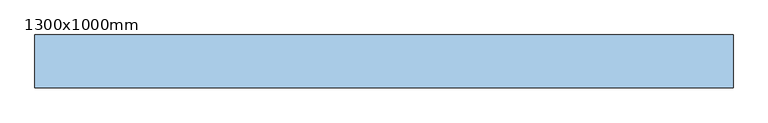
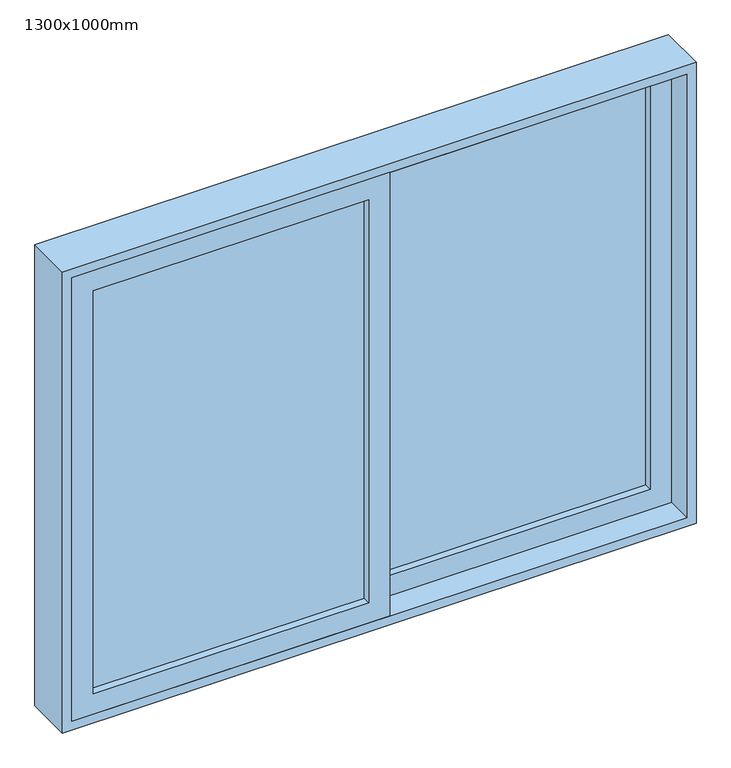
"""IFC4 building model written with IfcOpenShell, lengths in millimetres: window geometry, Janela de Correr - 2 Folhas : 1300x1000mm."""

import ifcopenshell
import ifcopenshell.guid

model = None  # the IFC model being written
_history = None  # IfcOwnerHistory: only IFC2X3 demands one
_inside = {}  # id of a spatial element -> (the spatial element, [elements in it])
_under = {}  # id of a project, library or spatial element -> (it, [spatial elements below it])
_declared = {}  # id of a project -> (the project, [libraries it declares])
_typed = {}  # id of a type object -> (the type object, [elements of that type])
_made_of = {}  # id of a material, layer set ... -> (it, [elements and type objects made of it])


def new_model(schema):
    """Start an empty IFC model of exactly this schema.

    Asked for "IFC4X3", IfcOpenShell would pick the latest addendum, in which some entities
    have other attributes; the version numbers below select the first issue.
    IFC2X3 requires an IfcOwnerHistory on every rooted entity: one is made here for all.
    """
    global model, _history
    if schema == "IFC4X3":
        model = ifcopenshell.file(schema_version=(4, 3, 0, 0))
    else:
        model = ifcopenshell.file(schema=schema)
    _inside.clear()
    _under.clear()
    _declared.clear()
    _typed.clear()
    _made_of.clear()
    _history = None
    if model.schema == "IFC2X3":
        org = make("IfcOrganization", Name="unknown")
        user = make(
            "IfcPersonAndOrganization",
            ThePerson=make("IfcPerson", FamilyName="unknown"),
            TheOrganization=org,
        )
        app = make(
            "IfcApplication",
            ApplicationDeveloper=org,
            Version="unknown",
            ApplicationFullName="unknown",
            ApplicationIdentifier="unknown",
        )
        _history = make(
            "IfcOwnerHistory",
            OwningUser=user,
            OwningApplication=app,
            ChangeAction="ADDED",
            CreationDate=0,
        )
    return model


def make(cls, **values):
    """One entity of the class cls with the attributes given. An attribute that is None is left unset."""
    return model.create_entity(
        cls, **{name: value for name, value in values.items() if value is not None}
    )


def rooted(cls, **values):
    """An entity with a GlobalId (a new one), such as an element, a storey or a relation."""
    return make(cls, GlobalId=ifcopenshell.guid.new(), OwnerHistory=_history, **values)


def si_unit(unit_type, name, prefix=None):
    """IfcSIUnit, for example si_unit("LENGTHUNIT", "METRE", prefix="MILLI")."""
    return make("IfcSIUnit", UnitType=unit_type, Prefix=prefix, Name=name)


def assignment(units):
    """IfcUnitAssignment: the units of a project."""
    return None if units is None else make("IfcUnitAssignment", Units=units)


def point(xyz):
    """IfcCartesianPoint."""
    return None if xyz is None else make("IfcCartesianPoint", Coordinates=xyz)


def direction(xyz):
    """IfcDirection."""
    return None if xyz is None else make("IfcDirection", DirectionRatios=xyz)


def frame(location, z_axis=None, x_axis=None):
    """IfcAxis2Placement3D, a coordinate frame: its origin and axes. An axis left out is left unset."""
    return make(
        "IfcAxis2Placement3D",
        Location=point(location),
        Axis=direction(z_axis),
        RefDirection=direction(x_axis),
    )


def origin():
    """The frame at (0, 0, 0) with its axes left unset."""
    return frame((0.0, 0.0, 0.0))


def place(relative_to, where):
    """IfcLocalPlacement: puts the frame where relative to a parent placement (None: the world)."""
    return make(
        "IfcLocalPlacement", PlacementRelTo=relative_to, RelativePlacement=where
    )


def context(
    kind, dimensions, precision=None, world=None, true_north=None, identifier=None
):
    """IfcGeometricRepresentationContext, for example the 3D "Model" context."""
    return make(
        "IfcGeometricRepresentationContext",
        ContextIdentifier=identifier,
        ContextType=kind,
        CoordinateSpaceDimension=dimensions,
        Precision=precision,
        WorldCoordinateSystem=world,
        TrueNorth=true_north,
    )


def project(units=None, contexts=None):
    """IfcProject with its units and contexts."""
    return rooted(
        "IfcProject",
        Name="project",
        RepresentationContexts=contexts,
        UnitsInContext=assignment(units),
    )


def spatial(cls, under=None, at=None, **own):
    """A site, building, storey or space (cls), placed at a placement, below another one or the project."""
    s = rooted(cls, ObjectPlacement=at, **own)
    if under is not None:
        _under.setdefault(under.id(), (under, []))[1].append(s)
    return s


def polyline(points):
    """IfcPolyline through the points."""
    return make("IfcPolyline", Points=[point(p) for p in points])


def outline(outer, holes=None, kind="AREA"):
    """IfcArbitraryClosedProfileDef: a profile drawn as a closed curve; with holes, ...WithVoids."""
    if holes is None:
        return make("IfcArbitraryClosedProfileDef", ProfileType=kind, OuterCurve=outer)
    return make(
        "IfcArbitraryProfileDefWithVoids",
        ProfileType=kind,
        OuterCurve=outer,
        InnerCurves=holes,
    )


def extrude(swept, where, along, depth):
    """IfcExtrudedAreaSolid: the profile swept, set in the frame where, extruded along a direction by depth."""
    return make(
        "IfcExtrudedAreaSolid",
        SweptArea=swept,
        Position=where,
        ExtrudedDirection=direction(along),
        Depth=depth,
    )


def shape(context_of_items, identifier, shape_type, items):
    """IfcShapeRepresentation: the items that make up one representation, for example the "Body"."""
    return make(
        "IfcShapeRepresentation",
        ContextOfItems=context_of_items,
        RepresentationIdentifier=identifier,
        RepresentationType=shape_type,
        Items=items,
    )


def source(mapping_origin, context_of_items, identifier, shape_type, items):
    """IfcRepresentationMap: a shape defined once, which mapped items show again and again."""
    return make(
        "IfcRepresentationMap",
        MappingOrigin=mapping_origin,
        MappedRepresentation=shape(context_of_items, identifier, shape_type, items),
    )


def transform(
    local_origin,
    x_axis=None,
    y_axis=None,
    z_axis=None,
    scale=None,
    scale2=None,
    scale3=None,
    uniform=True,
):
    """IfcCartesianTransformationOperator3D, or its non-uniform kind. x_axis, y_axis, z_axis: its Axis1, 2, 3."""
    if uniform:
        return make(
            "IfcCartesianTransformationOperator3D",
            Axis1=direction(x_axis),
            Axis2=direction(y_axis),
            LocalOrigin=point(local_origin),
            Scale=scale,
            Axis3=direction(z_axis),
        )
    return make(
        "IfcCartesianTransformationOperator3DnonUniform",
        Axis1=direction(x_axis),
        Axis2=direction(y_axis),
        LocalOrigin=point(local_origin),
        Scale=scale,
        Axis3=direction(z_axis),
        Scale2=scale2,
        Scale3=scale3,
    )


def mapped(mapping_source, mapping_target):
    """IfcMappedItem: shows the shape of a source again, moved by a transform."""
    return make(
        "IfcMappedItem", MappingSource=mapping_source, MappingTarget=mapping_target
    )


def made_of(thing, what):
    """Note that an element or type object is made of a material, layer set ...; save() writes the relation."""
    if what is not None:
        _made_of.setdefault(what.id(), (what, []))[1].append(thing)
    return thing


def element(
    cls,
    number,
    at=None,
    inside=None,
    cuts=None,
    type_object=None,
    material=None,
    context=None,
    identifier="Body",
    shape_type=None,
    held_by="IfcProductDefinitionShape",
    body=None,
    shapes=None,
    **own,
):
    """One element of the class cls, such as IfcWall. Its Tag is "e" and its number.

    at: its placement. inside: the storey or other place that contains it. cuts: it is an
    opening in that element (IfcRelVoidsElement). A single representation is given by context,
    identifier, shape_type and body (its items); several are given by shapes. held_by: the class
    of the entity that holds the representations. save() writes the other relations.
    """
    e = rooted(cls, Tag="e%d" % number, ObjectPlacement=at, **own)
    if body is not None:
        shapes = [shape(context, identifier, shape_type, body)]
    if shapes is not None:
        e.Representation = make(held_by, Representations=shapes)
    if inside is not None:
        _inside.setdefault(inside.id(), (inside, []))[1].append(e)
    if cuts is not None:
        rooted(
            "IfcRelVoidsElement", RelatingBuildingElement=cuts, RelatedOpeningElement=e
        )
    if type_object is not None:
        _typed.setdefault(type_object.id(), (type_object, []))[1].append(e)
    return made_of(e, material)


def aggregate(whole, parts):
    """IfcRelAggregates: a whole, such as a stair, and the parts it consists of."""
    return rooted("IfcRelAggregates", RelatingObject=whole, RelatedObjects=parts)


def save(model, path):
    """Write the relations noted so far, then the file.

    IfcRelAggregates (storeys below a building ...), IfcRelContainedInSpatialStructure (elements
    in a storey), IfcRelDefinesByType, IfcRelAssociatesMaterial and IfcRelDeclares: one each for
    every whole, place, type object, material and project.
    """
    for whole, parts in _under.values():
        aggregate(whole, parts)
    for where, things in _inside.values():
        rooted(
            "IfcRelContainedInSpatialStructure",
            RelatedElements=things,
            RelatingStructure=where,
        )
    for kind, things in _typed.values():
        rooted("IfcRelDefinesByType", RelatedObjects=things, RelatingType=kind)
    for what, things in _made_of.values():
        rooted("IfcRelAssociatesMaterial", RelatedObjects=things, RelatingMaterial=what)
    for by, libraries in _declared.values():
        rooted("IfcRelDeclares", RelatingContext=by, RelatedDefinitions=libraries)
    model.write(path)


def window_1300x1000mm_a11e05bc(model_context):
    return source(origin(), model_context, "Body", "SweptSolid", [
        extrude(outline(polyline([(-587.0, -44.6), (-22.0, -44.6), (-22.0, -56.6), (-587.0, -56.6), (-587.0, -44.6)])), frame((0.0, 0.0, 1263.0), z_axis=(0.0, 0.0, 1.0), x_axis=(1.0, 0.0, 0.0)), (0.0, 0.0, 1.0), 874.0),
        extrude(outline(polyline([(2181.0, 22.0), (2181.0, -631.0), (1219.0, -631.0), (1219.0, 22.0), (2181.0, 22.0)]), holes=[polyline([(2137.0, -22.0), (1263.0, -22.0), (1263.0, -587.0), (2137.0, -587.0), (2137.0, -22.0)])]), frame((0.0, -72.6, 0.0), z_axis=(0.0, 1.0, 0.0), x_axis=(0.0, 0.0, 1.0)), (0.0, 0.0, 1.0), 44.0),
        extrude(outline(polyline([(22.0, 9.4), (587.0, 9.4), (587.0, -2.6), (22.0, -2.6), (22.0, 9.4)])), frame((0.0, 0.0, 1263.0), z_axis=(0.0, 0.0, 1.0), x_axis=(1.0, 0.0, 0.0)), (0.0, 0.0, 1.0), 874.0),
        extrude(outline(polyline([(2181.0, -22.0), (1219.0, -22.0), (1219.0, 631.0), (2181.0, 631.0), (2181.0, -22.0)]), holes=[polyline([(2137.0, 22.0), (2137.0, 587.0), (1263.0, 587.0), (1263.0, 22.0), (2137.0, 22.0)])]), frame((0.0, -18.6, 0.0), z_axis=(0.0, 1.0, 0.0), x_axis=(0.0, 0.0, 1.0)), (0.0, 0.0, 1.0), 44.0),
        extrude(outline(polyline([(2200.0, -650.0), (1200.0, -650.0), (1200.0, 650.0), (2200.0, 650.0), (2200.0, -650.0)]), holes=[polyline([(2181.0, -631.0), (2181.0, 631.0), (1219.0, 631.0), (1219.0, -631.0), (2181.0, -631.0)])]), frame((0.0, -72.6, 0.0), z_axis=(0.0, 1.0, 0.0), x_axis=(0.0, 0.0, 1.0)), (0.0, 0.0, 1.0), 98.0),
    ])


if __name__ == "__main__":
    model = new_model("IFC4")
    model_context = context("Model", 3, world=origin())
    ifc_project = project(units=[si_unit("LENGTHUNIT", "METRE", prefix="MILLI")], contexts=[model_context])
    site = spatial("IfcSite", under=ifc_project)
    building = spatial("IfcBuilding", under=site)
    placement = place(None, origin())
    window_1300x1000mm_shape = window_1300x1000mm_a11e05bc(model_context)
    element("IfcWindow", 1, ObjectType="Janela de Correr - 2 Folhas : 1300x1000mm", at=placement, inside=building, context=model_context, shape_type="MappedRepresentation", body=[
        mapped(window_1300x1000mm_shape, transform((0.0, 0.0, 0.0), x_axis=(1.0, 0.0, 0.0), y_axis=(0.0, 1.0, 0.0), z_axis=(0.0, 0.0, 1.0))),
    ])
    save(model, "model.ifc")

# Revit data of these elements
# Project information
#   built-in parameter 1006321 = "01/01/2010"
#   built-in parameter 1006320 = "GDPProjetos.RVT"
#   built-in parameter 1006319 = "RAQUEL CANELLAS"
#   built-in parameter 1006318 = "Av. Treze de Maio 13 sl.1414  |Centro | Rio de Janeiro"
#   built-in parameter 1006317 = "GDP - Gerenciamento e Desenvolvimento de Projetos"
#   built-in parameter 1006316 = "100"
# Type "Janela de Correr - 2 Folhas : 1300x1000mm"
#   Type Mark = "J1"
#   SINAPI = ""
#   Módulo Básico M = 10.00 cm
#   Largura de Coordenação Modular CM = 130.00 cm
#   Altura de Coordenação Modular CM = 100.00 cm
#   Height = 100.00 cm
#   Altura Peitoril = 120.00 cm
#   Width = 130.00 cm
#   Largura Marco = 1.90 cm
#   Número de Módulos Básicos nM Largura = 13
#   Número de Módulos Básicos nM Altura = 10
#   Material Marco = Metal - Alumínio
#   Material Vidro = Vidro
#   Material Perfil = Metal - Alumínio
#   Construction Type = (empty or 0)
#   Description = (empty or 0)
#   Assembly Code = ""
#   Wall Closure = (empty or 0)
# Element 1 (IfcWindow, "Janela de Correr - 2 Folhas : 1300x1000mm")
#   Materials on its faces: "Metal - Alumínio", "Vidro", "Madeira - Faixa"
# Materials
#   "Metal - Alumínio": class "Metal", colour RGB 244 244 244, transparency 0
#   "Vidro": class "Vidro", colour RGB 230 230 230, transparency 0.75, Cost = 0
#   "Madeira - Faixa": class "Madeira", colour RGB 107 81 55, transparency 0, Cost = 0
